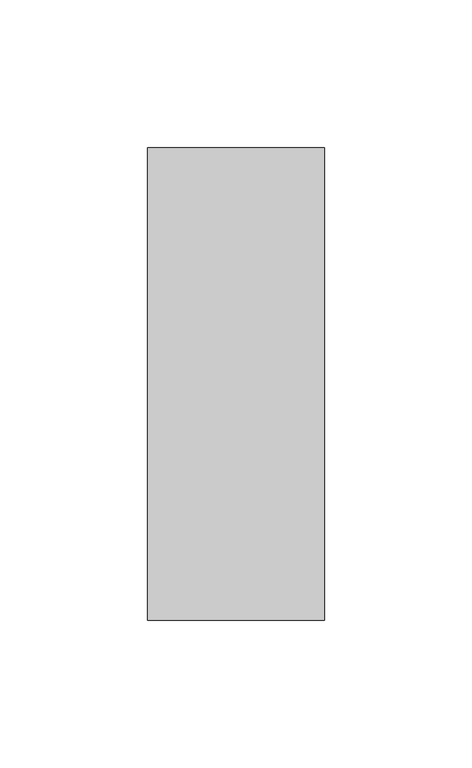
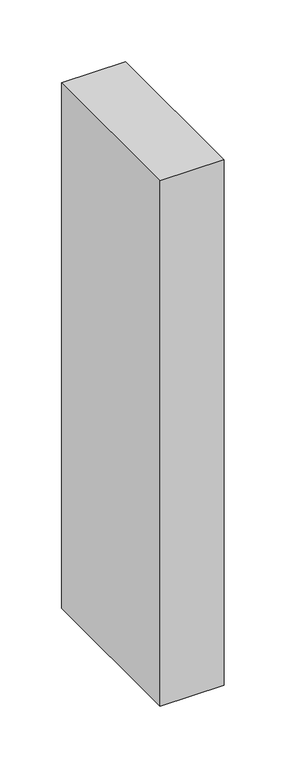
"""IFC4 building model written with IfcOpenShell, lengths in millimetres: column geometry, Madeira de lei-Coluna : Pontalete 6X16cm."""

import ifcopenshell
import ifcopenshell.guid

model = None  # the IFC model being written
_history = None  # IfcOwnerHistory: only IFC2X3 demands one
_inside = {}  # id of a spatial element -> (the spatial element, [elements in it])
_under = {}  # id of a project, library or spatial element -> (it, [spatial elements below it])
_declared = {}  # id of a project -> (the project, [libraries it declares])
_typed = {}  # id of a type object -> (the type object, [elements of that type])
_made_of = {}  # id of a material, layer set ... -> (it, [elements and type objects made of it])


def new_model(schema):
    """Start an empty IFC model of exactly this schema.

    Asked for "IFC4X3", IfcOpenShell would pick the latest addendum, in which some entities
    have other attributes; the version numbers below select the first issue.
    IFC2X3 requires an IfcOwnerHistory on every rooted entity: one is made here for all.
    """
    global model, _history
    if schema == "IFC4X3":
        model = ifcopenshell.file(schema_version=(4, 3, 0, 0))
    else:
        model = ifcopenshell.file(schema=schema)
    _inside.clear()
    _under.clear()
    _declared.clear()
    _typed.clear()
    _made_of.clear()
    _history = None
    if model.schema == "IFC2X3":
        org = make("IfcOrganization", Name="unknown")
        user = make(
            "IfcPersonAndOrganization",
            ThePerson=make("IfcPerson", FamilyName="unknown"),
            TheOrganization=org,
        )
        app = make(
            "IfcApplication",
            ApplicationDeveloper=org,
            Version="unknown",
            ApplicationFullName="unknown",
            ApplicationIdentifier="unknown",
        )
        _history = make(
            "IfcOwnerHistory",
            OwningUser=user,
            OwningApplication=app,
            ChangeAction="ADDED",
            CreationDate=0,
        )
    return model


def make(cls, **values):
    """One entity of the class cls with the attributes given. An attribute that is None is left unset."""
    return model.create_entity(
        cls, **{name: value for name, value in values.items() if value is not None}
    )


def rooted(cls, **values):
    """An entity with a GlobalId (a new one), such as an element, a storey or a relation."""
    return make(cls, GlobalId=ifcopenshell.guid.new(), OwnerHistory=_history, **values)


def si_unit(unit_type, name, prefix=None):
    """IfcSIUnit, for example si_unit("LENGTHUNIT", "METRE", prefix="MILLI")."""
    return make("IfcSIUnit", UnitType=unit_type, Prefix=prefix, Name=name)


def assignment(units):
    """IfcUnitAssignment: the units of a project."""
    return None if units is None else make("IfcUnitAssignment", Units=units)


def point(xyz):
    """IfcCartesianPoint."""
    return None if xyz is None else make("IfcCartesianPoint", Coordinates=xyz)


def direction(xyz):
    """IfcDirection."""
    return None if xyz is None else make("IfcDirection", DirectionRatios=xyz)


def frame(location, z_axis=None, x_axis=None):
    """IfcAxis2Placement3D, a coordinate frame: its origin and axes. An axis left out is left unset."""
    return make(
        "IfcAxis2Placement3D",
        Location=point(location),
        Axis=direction(z_axis),
        RefDirection=direction(x_axis),
    )


def origin():
    """The frame at (0, 0, 0) with its axes left unset."""
    return frame((0.0, 0.0, 0.0))


def place(relative_to, where):
    """IfcLocalPlacement: puts the frame where relative to a parent placement (None: the world)."""
    return make(
        "IfcLocalPlacement", PlacementRelTo=relative_to, RelativePlacement=where
    )


def context(
    kind, dimensions, precision=None, world=None, true_north=None, identifier=None
):
    """IfcGeometricRepresentationContext, for example the 3D "Model" context."""
    return make(
        "IfcGeometricRepresentationContext",
        ContextIdentifier=identifier,
        ContextType=kind,
        CoordinateSpaceDimension=dimensions,
        Precision=precision,
        WorldCoordinateSystem=world,
        TrueNorth=true_north,
    )


def project(units=None, contexts=None):
    """IfcProject with its units and contexts."""
    return rooted(
        "IfcProject",
        Name="project",
        RepresentationContexts=contexts,
        UnitsInContext=assignment(units),
    )


def spatial(cls, under=None, at=None, **own):
    """A site, building, storey or space (cls), placed at a placement, below another one or the project."""
    s = rooted(cls, ObjectPlacement=at, **own)
    if under is not None:
        _under.setdefault(under.id(), (under, []))[1].append(s)
    return s


def polyline(points):
    """IfcPolyline through the points."""
    return make("IfcPolyline", Points=[point(p) for p in points])


def outline(outer, holes=None, kind="AREA"):
    """IfcArbitraryClosedProfileDef: a profile drawn as a closed curve; with holes, ...WithVoids."""
    if holes is None:
        return make("IfcArbitraryClosedProfileDef", ProfileType=kind, OuterCurve=outer)
    return make(
        "IfcArbitraryProfileDefWithVoids",
        ProfileType=kind,
        OuterCurve=outer,
        InnerCurves=holes,
    )


def extrude(swept, where, along, depth):
    """IfcExtrudedAreaSolid: the profile swept, set in the frame where, extruded along a direction by depth."""
    return make(
        "IfcExtrudedAreaSolid",
        SweptArea=swept,
        Position=where,
        ExtrudedDirection=direction(along),
        Depth=depth,
    )


def shape(context_of_items, identifier, shape_type, items):
    """IfcShapeRepresentation: the items that make up one representation, for example the "Body"."""
    return make(
        "IfcShapeRepresentation",
        ContextOfItems=context_of_items,
        RepresentationIdentifier=identifier,
        RepresentationType=shape_type,
        Items=items,
    )


def source(mapping_origin, context_of_items, identifier, shape_type, items):
    """IfcRepresentationMap: a shape defined once, which mapped items show again and again."""
    return make(
        "IfcRepresentationMap",
        MappingOrigin=mapping_origin,
        MappedRepresentation=shape(context_of_items, identifier, shape_type, items),
    )


def transform(
    local_origin,
    x_axis=None,
    y_axis=None,
    z_axis=None,
    scale=None,
    scale2=None,
    scale3=None,
    uniform=True,
):
    """IfcCartesianTransformationOperator3D, or its non-uniform kind. x_axis, y_axis, z_axis: its Axis1, 2, 3."""
    if uniform:
        return make(
            "IfcCartesianTransformationOperator3D",
            Axis1=direction(x_axis),
            Axis2=direction(y_axis),
            LocalOrigin=point(local_origin),
            Scale=scale,
            Axis3=direction(z_axis),
        )
    return make(
        "IfcCartesianTransformationOperator3DnonUniform",
        Axis1=direction(x_axis),
        Axis2=direction(y_axis),
        LocalOrigin=point(local_origin),
        Scale=scale,
        Axis3=direction(z_axis),
        Scale2=scale2,
        Scale3=scale3,
    )


def mapped(mapping_source, mapping_target):
    """IfcMappedItem: shows the shape of a source again, moved by a transform."""
    return make(
        "IfcMappedItem", MappingSource=mapping_source, MappingTarget=mapping_target
    )


def made_of(thing, what):
    """Note that an element or type object is made of a material, layer set ...; save() writes the relation."""
    if what is not None:
        _made_of.setdefault(what.id(), (what, []))[1].append(thing)
    return thing


def element(
    cls,
    number,
    at=None,
    inside=None,
    cuts=None,
    type_object=None,
    material=None,
    context=None,
    identifier="Body",
    shape_type=None,
    held_by="IfcProductDefinitionShape",
    body=None,
    shapes=None,
    **own,
):
    """One element of the class cls, such as IfcWall. Its Tag is "e" and its number.

    at: its placement. inside: the storey or other place that contains it. cuts: it is an
    opening in that element (IfcRelVoidsElement). A single representation is given by context,
    identifier, shape_type and body (its items); several are given by shapes. held_by: the class
    of the entity that holds the representations. save() writes the other relations.
    """
    e = rooted(cls, Tag="e%d" % number, ObjectPlacement=at, **own)
    if body is not None:
        shapes = [shape(context, identifier, shape_type, body)]
    if shapes is not None:
        e.Representation = make(held_by, Representations=shapes)
    if inside is not None:
        _inside.setdefault(inside.id(), (inside, []))[1].append(e)
    if cuts is not None:
        rooted(
            "IfcRelVoidsElement", RelatingBuildingElement=cuts, RelatedOpeningElement=e
        )
    if type_object is not None:
        _typed.setdefault(type_object.id(), (type_object, []))[1].append(e)
    return made_of(e, material)


def aggregate(whole, parts):
    """IfcRelAggregates: a whole, such as a stair, and the parts it consists of."""
    return rooted("IfcRelAggregates", RelatingObject=whole, RelatedObjects=parts)


def save(model, path):
    """Write the relations noted so far, then the file.

    IfcRelAggregates (storeys below a building ...), IfcRelContainedInSpatialStructure (elements
    in a storey), IfcRelDefinesByType, IfcRelAssociatesMaterial and IfcRelDeclares: one each for
    every whole, place, type object, material and project.
    """
    for whole, parts in _under.values():
        aggregate(whole, parts)
    for where, things in _inside.values():
        rooted(
            "IfcRelContainedInSpatialStructure",
            RelatedElements=things,
            RelatingStructure=where,
        )
    for kind, things in _typed.values():
        rooted("IfcRelDefinesByType", RelatedObjects=things, RelatingType=kind)
    for what, things in _made_of.values():
        rooted("IfcRelAssociatesMaterial", RelatedObjects=things, RelatingMaterial=what)
    for by, libraries in _declared.values():
        rooted("IfcRelDeclares", RelatingContext=by, RelatedDefinitions=libraries)
    model.write(path)


def column_d0cf395a(model_context):
    return source(origin(), model_context, "Body", "SweptSolid", [
        extrude(outline(polyline([(30.0, 80.0), (30.0, -80.0), (-30.0, -80.0), (-30.0, 80.0), (30.0, 80.0)])), frame((0.0, 0.0, 6710.0), z_axis=(0.0, 0.0, 1.0), x_axis=(1.0, 0.0, 0.0)), (0.0, 0.0, 1.0), 520.0),
    ])


if __name__ == "__main__":
    model = new_model("IFC4")
    model_context = context("Model", 3, world=origin())
    ifc_project = project(units=[si_unit("LENGTHUNIT", "METRE", prefix="MILLI")], contexts=[model_context])
    site = spatial("IfcSite", under=ifc_project)
    building = spatial("IfcBuilding", under=site)
    placement = place(None, origin())
    column_shape = column_d0cf395a(model_context)
    element("IfcColumn", 1, ObjectType="Madeira de lei-Coluna : Pontalete 6X16cm", at=placement, inside=building, context=model_context, shape_type="MappedRepresentation", body=[
        mapped(column_shape, transform((0.0, 0.0, 0.0), x_axis=(1.0, 0.0, 0.0), y_axis=(0.0, 1.0, 0.0), z_axis=(0.0, 0.0, 1.0))),
    ])
    save(model, "model.ifc")

# Revit data of these elements
# Type "Madeira de lei-Coluna : Pontalete 6X16cm"
#   A = 0.01952 m²
#   b = 0.06 m
#   d = 0.16 m
#   Structural Material [instance default] = none
#   Assembly Code = ""
# Element 1 (IfcColumn, "Madeira de lei-Coluna : Pontalete 6X16cm")
#   Structural Material = .MADEIRAMENTO
#   Materials on its faces: ".MADEIRAMENTO"
# Materials
#   ".MADEIRAMENTO": class ".CC_MADEIRAS", colour RGB 212 179 113, transparency 0, Cost = 0
